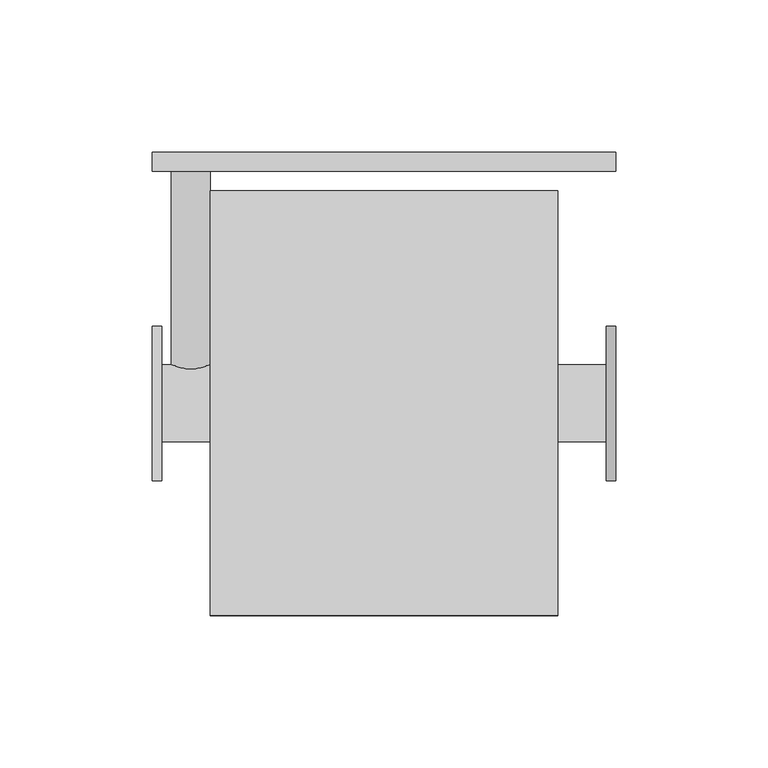
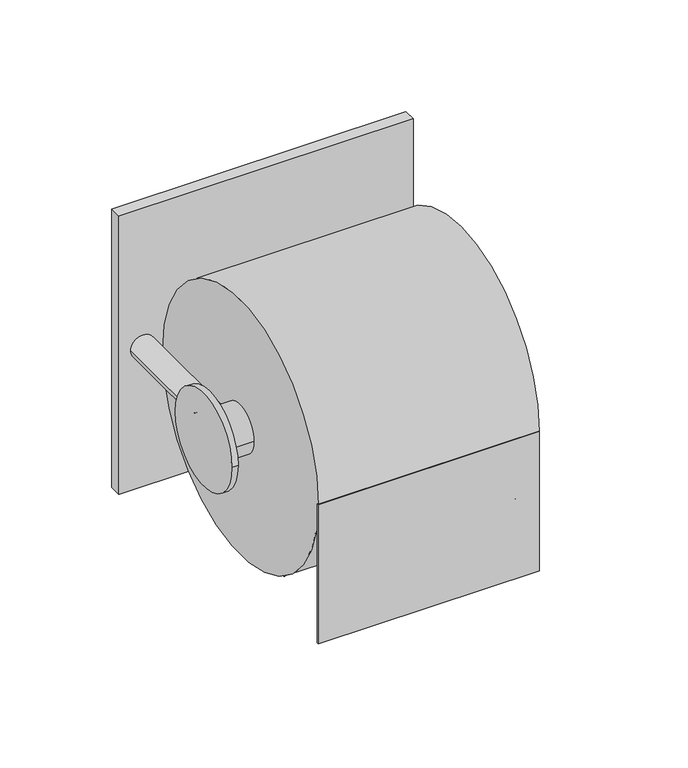
"""IFC4 building model written with IfcOpenShell, lengths in millimetres: proxy geometry, Dispenser, Toilet Paper - NON-COLLECTUS : -."""

from ifc_helpers import new_model, si_unit, point, frame, frame_2d, origin, origin_with_axes, place, context, project, spatial, polyline, circle_curve, trimmed, segment, composite_curve, outline, extrude, source, transform, mapped, element, save


def specialty_equipment_c18e75ea(model_context):
    return source(origin(), model_context, "Body", "SweptSolid", [
        extrude(outline(polyline([(57.15, -151.5070313), (57.15, -152.4), (-57.15, -152.4), (-57.15, -151.5070313), (57.15, -151.5070313)])), origin_with_axes(), (0.0, 0.0, 1.0), 76.2),
        extrude(outline(composite_curve([segment(trimmed(circle_curve(frame_2d((-82.55, 76.2)), 69.85), [point((-152.4, 76.2))], [point((-12.7, 76.2))], False, "CARTESIAN"), True, "CONTINUOUS"), segment(trimmed(circle_curve(frame_2d((-82.55, 76.2)), 69.85), [point((-12.7, 76.2))], [point((-152.4, 76.2))], False, "CARTESIAN"), True, "CONTINUOUS")], self_intersect=False)), frame((-57.15, 0.0, 0.0), z_axis=(1.0, 0.0, 0.0), x_axis=(0.0, 1.0, 0.0)), (0.0, 0.0, 1.0), 114.3),
        extrude(outline(composite_curve([segment(trimmed(circle_curve(frame_2d((-82.55, 76.2)), 25.4), [point((-107.95, 76.2))], [point((-57.15, 76.2))], False, "CARTESIAN"), True, "CONTINUOUS"), segment(trimmed(circle_curve(frame_2d((-82.55, 76.2)), 25.4), [point((-57.15, 76.2))], [point((-107.95, 76.2))], False, "CARTESIAN"), True, "CONTINUOUS")], self_intersect=False)), frame((73.025, 0.0, 0.0), z_axis=(1.0, 0.0, 0.0), x_axis=(0.0, 1.0, 0.0)), (0.0, 0.0, 1.0), 3.175),
        extrude(outline(composite_curve([segment(trimmed(circle_curve(frame_2d((-82.55, 76.2)), 25.4), [point((-107.95, 76.2))], [point((-57.15, 76.2))], False, "CARTESIAN"), True, "CONTINUOUS"), segment(trimmed(circle_curve(frame_2d((-82.55, 76.2)), 25.4), [point((-57.15, 76.2))], [point((-107.95, 76.2))], False, "CARTESIAN"), True, "CONTINUOUS")], self_intersect=False)), frame((-76.2, 0.0, 0.0), z_axis=(1.0, 0.0, 0.0), x_axis=(0.0, 1.0, 0.0)), (0.0, 0.0, 1.0), 3.175),
        extrude(outline(composite_curve([segment(trimmed(circle_curve(frame_2d((-82.55, 76.2)), 12.7), [point((-95.25, 76.2))], [point((-69.85, 76.2))], False, "CARTESIAN"), True, "CONTINUOUS"), segment(trimmed(circle_curve(frame_2d((-82.55, 76.2)), 12.7), [point((-69.85, 76.2))], [point((-95.25, 76.2))], False, "CARTESIAN"), True, "CONTINUOUS")], self_intersect=False)), frame((-76.2, 0.0, 0.0), z_axis=(1.0, 0.0, 0.0), x_axis=(0.0, 1.0, 0.0)), (0.0, 0.0, 1.0), 152.4),
        extrude(outline(composite_curve([segment(trimmed(circle_curve(frame_2d((76.2, -63.5)), 6.35), [point((76.2, -69.85))], [point((76.2, -57.15))], False, "CARTESIAN"), True, "CONTINUOUS"), segment(trimmed(circle_curve(frame_2d((76.2, -63.5)), 6.35), [point((76.2, -57.15))], [point((76.2, -69.85))], False, "CARTESIAN"), True, "CONTINUOUS")], self_intersect=False)), frame((0.0, -82.55, 0.0), z_axis=(0.0, 1.0, 0.0), x_axis=(0.0, 0.0, 1.0)), (0.0, 0.0, 1.0), 82.55),
        extrude(outline(polyline([(76.2, -6.35), (-76.2, -6.35), (-76.2, 0.0), (76.2, 0.0), (76.2, -6.35)])), origin_with_axes(), (0.0, 0.0, 1.0), 152.4),
    ])


if __name__ == "__main__":
    model = new_model("IFC4")
    model_context = context("Model", 3, world=origin())
    ifc_project = project(units=[si_unit("LENGTHUNIT", "METRE", prefix="MILLI")], contexts=[model_context])
    site = spatial("IfcSite", under=ifc_project)
    building = spatial("IfcBuilding", under=site)
    placement = place(None, origin())
    specialty_equipment_shape = specialty_equipment_c18e75ea(model_context)
    element("IfcBuildingElementProxy", 1, Name="Dispenser, Toilet Paper - NON-COLLECTUS : -", ObjectType="Dispenser, Toilet Paper - NON-COLLECTUS : -", at=placement, inside=building, context=model_context, shape_type="MappedRepresentation", body=[
        mapped(specialty_equipment_shape, transform((0.0, 0.0, 0.0), x_axis=(1.0, 0.0, 0.0), y_axis=(0.0, 1.0, 0.0), z_axis=(0.0, 0.0, 1.0))),
    ])
    save(model, "model.ifc")

# Revit data of these elements
# Type "Dispenser, Toilet Paper - NON-COLLECTUS : -"
#   External ID [instance default] = ""
#   Width = 152.4 mm
#   Height = 152.4 mm
#   Depth = 152.4 mm
#   Material = White
#   Default Elevation = 0
# Element 1 (IfcBuildingElementProxy, "Dispenser, Toilet Paper - NON-COLLECTUS : -")
#   Materials on its faces: "White"
# Materials
#   "White": class "Generic", colour RGB 255 255 255, transparency 0, Cost = 0
